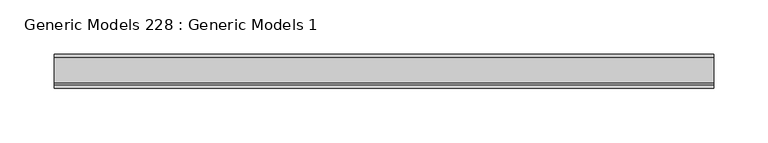
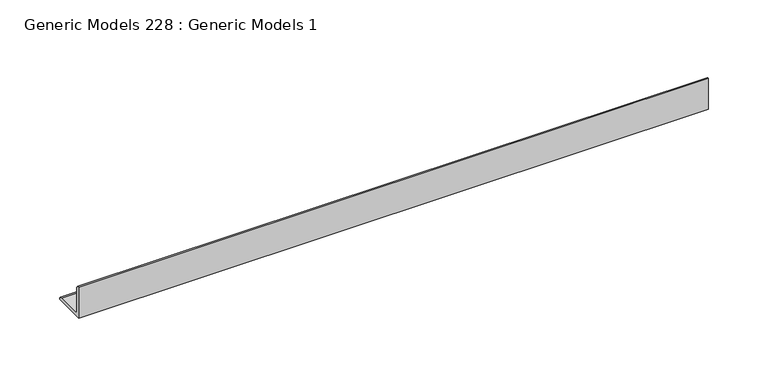
"""IFC4 building model written with IfcOpenShell, lengths in millimetres: proxy geometry, Generic Models 228 : Generic Models 1."""

import ifcopenshell
import ifcopenshell.guid

model = None  # the IFC model being written
_history = None  # IfcOwnerHistory: only IFC2X3 demands one
_inside = {}  # id of a spatial element -> (the spatial element, [elements in it])
_under = {}  # id of a project, library or spatial element -> (it, [spatial elements below it])
_declared = {}  # id of a project -> (the project, [libraries it declares])
_typed = {}  # id of a type object -> (the type object, [elements of that type])
_made_of = {}  # id of a material, layer set ... -> (it, [elements and type objects made of it])


def new_model(schema):
    """Start an empty IFC model of exactly this schema.

    Asked for "IFC4X3", IfcOpenShell would pick the latest addendum, in which some entities
    have other attributes; the version numbers below select the first issue.
    IFC2X3 requires an IfcOwnerHistory on every rooted entity: one is made here for all.
    """
    global model, _history
    if schema == "IFC4X3":
        model = ifcopenshell.file(schema_version=(4, 3, 0, 0))
    else:
        model = ifcopenshell.file(schema=schema)
    _inside.clear()
    _under.clear()
    _declared.clear()
    _typed.clear()
    _made_of.clear()
    _history = None
    if model.schema == "IFC2X3":
        org = make("IfcOrganization", Name="unknown")
        user = make(
            "IfcPersonAndOrganization",
            ThePerson=make("IfcPerson", FamilyName="unknown"),
            TheOrganization=org,
        )
        app = make(
            "IfcApplication",
            ApplicationDeveloper=org,
            Version="unknown",
            ApplicationFullName="unknown",
            ApplicationIdentifier="unknown",
        )
        _history = make(
            "IfcOwnerHistory",
            OwningUser=user,
            OwningApplication=app,
            ChangeAction="ADDED",
            CreationDate=0,
        )
    return model


def make(cls, **values):
    """One entity of the class cls with the attributes given. An attribute that is None is left unset."""
    return model.create_entity(
        cls, **{name: value for name, value in values.items() if value is not None}
    )


def rooted(cls, **values):
    """An entity with a GlobalId (a new one), such as an element, a storey or a relation."""
    return make(cls, GlobalId=ifcopenshell.guid.new(), OwnerHistory=_history, **values)


def si_unit(unit_type, name, prefix=None):
    """IfcSIUnit, for example si_unit("LENGTHUNIT", "METRE", prefix="MILLI")."""
    return make("IfcSIUnit", UnitType=unit_type, Prefix=prefix, Name=name)


def assignment(units):
    """IfcUnitAssignment: the units of a project."""
    return None if units is None else make("IfcUnitAssignment", Units=units)


def point(xyz):
    """IfcCartesianPoint."""
    return None if xyz is None else make("IfcCartesianPoint", Coordinates=xyz)


def direction(xyz):
    """IfcDirection."""
    return None if xyz is None else make("IfcDirection", DirectionRatios=xyz)


def frame(location, z_axis=None, x_axis=None):
    """IfcAxis2Placement3D, a coordinate frame: its origin and axes. An axis left out is left unset."""
    return make(
        "IfcAxis2Placement3D",
        Location=point(location),
        Axis=direction(z_axis),
        RefDirection=direction(x_axis),
    )


def frame_2d(location, x_axis=None):
    """IfcAxis2Placement2D, a coordinate frame in the plane: its origin and x axis."""
    return make(
        "IfcAxis2Placement2D", Location=point(location), RefDirection=direction(x_axis)
    )


def origin():
    """The frame at (0, 0, 0) with its axes left unset."""
    return frame((0.0, 0.0, 0.0))


def place(relative_to, where):
    """IfcLocalPlacement: puts the frame where relative to a parent placement (None: the world)."""
    return make(
        "IfcLocalPlacement", PlacementRelTo=relative_to, RelativePlacement=where
    )


def context(
    kind, dimensions, precision=None, world=None, true_north=None, identifier=None
):
    """IfcGeometricRepresentationContext, for example the 3D "Model" context."""
    return make(
        "IfcGeometricRepresentationContext",
        ContextIdentifier=identifier,
        ContextType=kind,
        CoordinateSpaceDimension=dimensions,
        Precision=precision,
        WorldCoordinateSystem=world,
        TrueNorth=true_north,
    )


def project(units=None, contexts=None):
    """IfcProject with its units and contexts."""
    return rooted(
        "IfcProject",
        Name="project",
        RepresentationContexts=contexts,
        UnitsInContext=assignment(units),
    )


def spatial(cls, under=None, at=None, **own):
    """A site, building, storey or space (cls), placed at a placement, below another one or the project."""
    s = rooted(cls, ObjectPlacement=at, **own)
    if under is not None:
        _under.setdefault(under.id(), (under, []))[1].append(s)
    return s


def polyline(points):
    """IfcPolyline through the points."""
    return make("IfcPolyline", Points=[point(p) for p in points])


def circle_curve(where, radius):
    """IfcCircle in the frame where."""
    return make("IfcCircle", Position=where, Radius=radius)


def trimmed(basis, trim1, trim2, sense, master):
    """IfcTrimmedCurve: the piece of a basis curve between two trims."""
    return make(
        "IfcTrimmedCurve",
        BasisCurve=basis,
        Trim1=trim1,
        Trim2=trim2,
        SenseAgreement=sense,
        MasterRepresentation=master,
    )


def segment(curve, same_sense, transition):
    """IfcCompositeCurveSegment."""
    return make(
        "IfcCompositeCurveSegment",
        Transition=transition,
        SameSense=same_sense,
        ParentCurve=curve,
    )


def composite_curve(segments, self_intersect=None):
    """IfcCompositeCurve: segments joined end to end."""
    return make("IfcCompositeCurve", Segments=segments, SelfIntersect=self_intersect)


def outline(outer, holes=None, kind="AREA"):
    """IfcArbitraryClosedProfileDef: a profile drawn as a closed curve; with holes, ...WithVoids."""
    if holes is None:
        return make("IfcArbitraryClosedProfileDef", ProfileType=kind, OuterCurve=outer)
    return make(
        "IfcArbitraryProfileDefWithVoids",
        ProfileType=kind,
        OuterCurve=outer,
        InnerCurves=holes,
    )


def extrude(swept, where, along, depth):
    """IfcExtrudedAreaSolid: the profile swept, set in the frame where, extruded along a direction by depth."""
    return make(
        "IfcExtrudedAreaSolid",
        SweptArea=swept,
        Position=where,
        ExtrudedDirection=direction(along),
        Depth=depth,
    )


def shape(context_of_items, identifier, shape_type, items):
    """IfcShapeRepresentation: the items that make up one representation, for example the "Body"."""
    return make(
        "IfcShapeRepresentation",
        ContextOfItems=context_of_items,
        RepresentationIdentifier=identifier,
        RepresentationType=shape_type,
        Items=items,
    )


def source(mapping_origin, context_of_items, identifier, shape_type, items):
    """IfcRepresentationMap: a shape defined once, which mapped items show again and again."""
    return make(
        "IfcRepresentationMap",
        MappingOrigin=mapping_origin,
        MappedRepresentation=shape(context_of_items, identifier, shape_type, items),
    )


def transform(
    local_origin,
    x_axis=None,
    y_axis=None,
    z_axis=None,
    scale=None,
    scale2=None,
    scale3=None,
    uniform=True,
):
    """IfcCartesianTransformationOperator3D, or its non-uniform kind. x_axis, y_axis, z_axis: its Axis1, 2, 3."""
    if uniform:
        return make(
            "IfcCartesianTransformationOperator3D",
            Axis1=direction(x_axis),
            Axis2=direction(y_axis),
            LocalOrigin=point(local_origin),
            Scale=scale,
            Axis3=direction(z_axis),
        )
    return make(
        "IfcCartesianTransformationOperator3DnonUniform",
        Axis1=direction(x_axis),
        Axis2=direction(y_axis),
        LocalOrigin=point(local_origin),
        Scale=scale,
        Axis3=direction(z_axis),
        Scale2=scale2,
        Scale3=scale3,
    )


def mapped(mapping_source, mapping_target):
    """IfcMappedItem: shows the shape of a source again, moved by a transform."""
    return make(
        "IfcMappedItem", MappingSource=mapping_source, MappingTarget=mapping_target
    )


def made_of(thing, what):
    """Note that an element or type object is made of a material, layer set ...; save() writes the relation."""
    if what is not None:
        _made_of.setdefault(what.id(), (what, []))[1].append(thing)
    return thing


def element(
    cls,
    number,
    at=None,
    inside=None,
    cuts=None,
    type_object=None,
    material=None,
    context=None,
    identifier="Body",
    shape_type=None,
    held_by="IfcProductDefinitionShape",
    body=None,
    shapes=None,
    **own,
):
    """One element of the class cls, such as IfcWall. Its Tag is "e" and its number.

    at: its placement. inside: the storey or other place that contains it. cuts: it is an
    opening in that element (IfcRelVoidsElement). A single representation is given by context,
    identifier, shape_type and body (its items); several are given by shapes. held_by: the class
    of the entity that holds the representations. save() writes the other relations.
    """
    e = rooted(cls, Tag="e%d" % number, ObjectPlacement=at, **own)
    if body is not None:
        shapes = [shape(context, identifier, shape_type, body)]
    if shapes is not None:
        e.Representation = make(held_by, Representations=shapes)
    if inside is not None:
        _inside.setdefault(inside.id(), (inside, []))[1].append(e)
    if cuts is not None:
        rooted(
            "IfcRelVoidsElement", RelatingBuildingElement=cuts, RelatedOpeningElement=e
        )
    if type_object is not None:
        _typed.setdefault(type_object.id(), (type_object, []))[1].append(e)
    return made_of(e, material)


def aggregate(whole, parts):
    """IfcRelAggregates: a whole, such as a stair, and the parts it consists of."""
    return rooted("IfcRelAggregates", RelatingObject=whole, RelatedObjects=parts)


def save(model, path):
    """Write the relations noted so far, then the file.

    IfcRelAggregates (storeys below a building ...), IfcRelContainedInSpatialStructure (elements
    in a storey), IfcRelDefinesByType, IfcRelAssociatesMaterial and IfcRelDeclares: one each for
    every whole, place, type object, material and project.
    """
    for whole, parts in _under.values():
        aggregate(whole, parts)
    for where, things in _inside.values():
        rooted(
            "IfcRelContainedInSpatialStructure",
            RelatedElements=things,
            RelatingStructure=where,
        )
    for kind, things in _typed.values():
        rooted("IfcRelDefinesByType", RelatedObjects=things, RelatingType=kind)
    for what, things in _made_of.values():
        rooted("IfcRelAssociatesMaterial", RelatedObjects=things, RelatingMaterial=what)
    for by, libraries in _declared.values():
        rooted("IfcRelDeclares", RelatingContext=by, RelatedDefinitions=libraries)
    model.write(path)


def generic_models_228_generic_models_1_053e8907(model_context):
    return source(origin(), model_context, "Body", "SweptSolid", [
        extrude(outline(composite_curve([segment(polyline([(592.1375, 4235.45), (592.1375, 4267.2)]), True, "CONTINUOUS"), segment(trimmed(circle_curve(frame_2d((592.1375, 4264.025)), 3.175), [point((592.1375, 4267.2))], [point((595.3125, 4264.025))], False, "CARTESIAN"), True, "CONTINUOUS"), segment(polyline([(595.3125, 4264.025), (595.3125, 4240.2125)]), True, "CONTINUOUS"), segment(trimmed(circle_curve(frame_2d((596.9, 4240.2125)), 1.5875), [point((595.3125, 4240.2125))], [point((596.9, 4238.625))], True, "CARTESIAN"), True, "CONTINUOUS"), segment(polyline([(596.9, 4238.625), (620.7125, 4238.625)]), True, "CONTINUOUS"), segment(trimmed(circle_curve(frame_2d((620.7125, 4235.45)), 3.175), [point((620.7125, 4238.625))], [point((623.8875, 4235.45))], False, "CARTESIAN"), True, "CONTINUOUS"), segment(polyline([(623.8875, 4235.45), (592.1375, 4235.45)]), True, "CONTINUOUS")], self_intersect=False)), frame((46753.4625, 0.0, 0.0), z_axis=(1.0, 0.0, 0.0), x_axis=(0.0, 1.0, 0.0)), (0.0, 0.0, 1.0), 609.6),
    ])


if __name__ == "__main__":
    model = new_model("IFC4")
    model_context = context("Model", 3, world=origin())
    ifc_project = project(units=[si_unit("LENGTHUNIT", "METRE", prefix="MILLI")], contexts=[model_context])
    site = spatial("IfcSite", under=ifc_project)
    building = spatial("IfcBuilding", under=site)
    placement = place(None, origin())
    generic_models_228_generic_models_1_shape = generic_models_228_generic_models_1_053e8907(model_context)
    element("IfcBuildingElementProxy", 1, Name="Generic Models 228 : Generic Models 1", ObjectType="Generic Models 228 : Generic Models 1", at=placement, inside=building, context=model_context, shape_type="MappedRepresentation", body=[
        mapped(generic_models_228_generic_models_1_shape, transform((0.0, 0.0, 0.0), x_axis=(1.0, 0.0, 0.0), y_axis=(0.0, 1.0, 0.0), z_axis=(0.0, 0.0, 1.0))),
    ])
    save(model, "model.ifc")

# Revit data of these elements
# Element 1 (IfcBuildingElementProxy, "Generic Models 228 : Generic Models 1")
#   Materials on its faces: "BULKHEAD FRAME WORK"
# Materials
#   "BULKHEAD FRAME WORK": class "Metal", colour RGB 189 187 185, transparency 0, Description = "Structural steel 50ksi", Cost = 0
